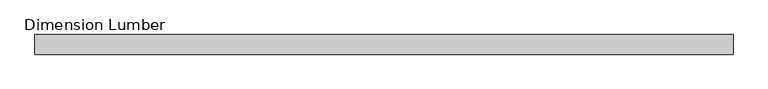
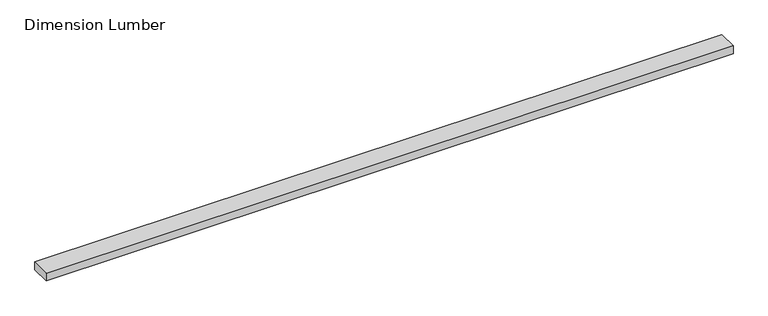
"""IFC4 building model written with IfcOpenShell, lengths in millimetres: beam geometry, Dimension Lumber : Top Supporting Lumbers."""

from ifc_helpers import new_model, si_unit, frame, origin, place, context, project, spatial, polyline, outline, extrude, source, transform, mapped, element, save


def dimension_lumber_0ba03532(model_context):
    return source(origin(), model_context, "Body", "SweptSolid", [
        extrude(outline(polyline([(1590.9128229, 44.45), (1590.9128229, -44.45), (-1571.3871771, -44.45), (-1571.3871771, 44.45), (1590.9128229, 44.45)])), frame((0.0, 0.0, -19.05), z_axis=(0.0, 0.0, 1.0), x_axis=(1.0, 0.0, 0.0)), (0.0, 0.0, 1.0), 38.1),
    ])


if __name__ == "__main__":
    model = new_model("IFC4")
    model_context = context("Model", 3, world=origin())
    ifc_project = project(units=[si_unit("LENGTHUNIT", "METRE", prefix="MILLI")], contexts=[model_context])
    site = spatial("IfcSite", under=ifc_project)
    building = spatial("IfcBuilding", under=site)
    placement = place(None, origin())
    dimension_lumber_shape = dimension_lumber_0ba03532(model_context)
    element("IfcBeam", 1, ObjectType="Dimension Lumber : Top Supporting Lumbers", at=placement, inside=building, context=model_context, shape_type="MappedRepresentation", body=[
        mapped(dimension_lumber_shape, transform((0.0, 0.0, 0.0), x_axis=(1.0, 0.0, 0.0), y_axis=(0.0, 1.0, 0.0), z_axis=(0.0, 0.0, 1.0))),
    ])
    save(model, "model.ifc")

# Revit data of these elements
# Type "Dimension Lumber : Top Supporting Lumbers"
#   Assembly Code = "B10"
#   A = 0.0364583 SF
#   Length [instance default] = 5' - 0"
#   b = 0' - 3 1/2"
#   d = 0' - 1 1/2"
#   Structural Material [instance default] = Softwood, Lumber
# Element 1 (IfcBeam, "Dimension Lumber : Top Supporting Lumbers")
#   Structural Material = Douglas Fir #2
#   Materials on its faces: "Douglas Fir #2"
# Materials
#   "Softwood, Lumber": class "Wood", colour RGB 223 192 134, transparency 0, Description = "Pinus Echinata", Cost = 0
#   "Douglas Fir #2": class "Wood", colour RGB 223 192 134, transparency 0, Description = "Pinus Echinata", Cost = 0
